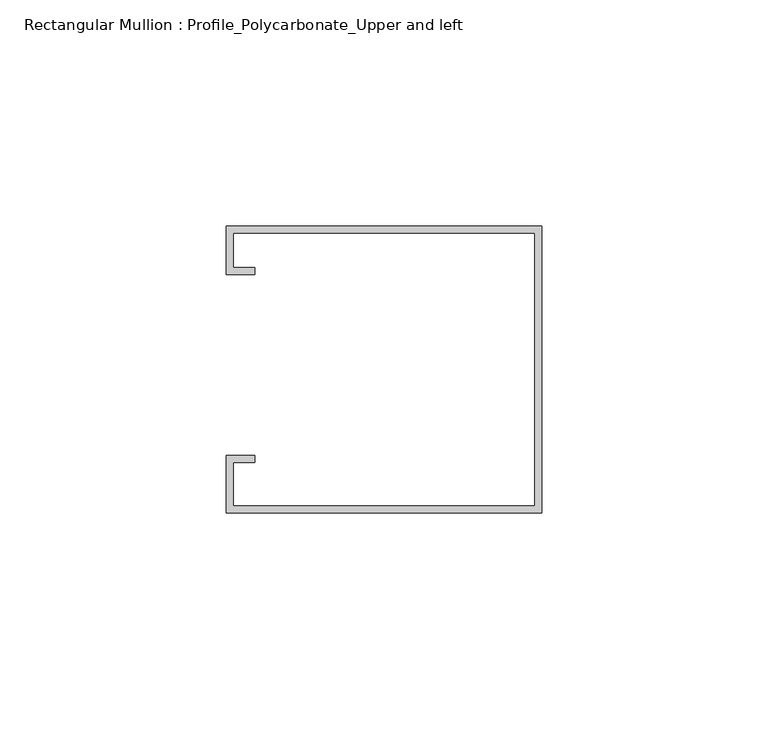
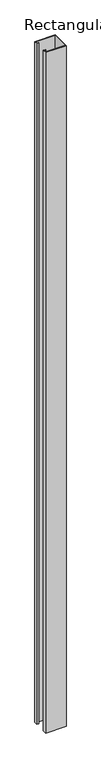
"""IFC4 building model written with IfcOpenShell, lengths in millimetres: member geometry, Rectangular Mullion : Profile_Polycarbonate_Upper and left."""

from ifc_helpers import new_model, si_unit, frame, origin, place, context, project, spatial, polyline, outline, extrude, source, transform, mapped, element, save


def rectangular_mullion_profile_polycarbonate_upper_and_left_a3cdb98e(model_context):
    return source(origin(), model_context, "Body", "SweptSolid", [
        extrude(outline(polyline([(0.0, -32.7), (-69.85, -32.7), (-69.85, -20.0), (-63.5, -20.0), (-63.5, -21.5875), (-68.2625, -21.5875), (-68.2625, -31.1125), (-1.5875, -31.1125), (-1.5875, 29.2125), (-68.2625, 29.2125), (-68.2625, 21.5875), (-63.5, 21.5875), (-63.5, 20.0), (-69.85, 20.0), (-69.85, 30.8), (0.0, 30.8), (0.0, -32.7)])), frame((0.0, 0.0, -2461.6132885), z_axis=(0.0, 0.0, 1.0), x_axis=(1.0, 0.0, 0.0)), (0.0, 0.0, 1.0), 2461.6132885),
    ])


if __name__ == "__main__":
    model = new_model("IFC4")
    model_context = context("Model", 3, world=origin())
    ifc_project = project(units=[si_unit("LENGTHUNIT", "METRE", prefix="MILLI")], contexts=[model_context])
    site = spatial("IfcSite", under=ifc_project)
    building = spatial("IfcBuilding", under=site)
    placement = place(None, origin())
    rectangular_mullion_profile_polycarbonate_upper_and_left_shape = rectangular_mullion_profile_polycarbonate_upper_and_left_a3cdb98e(model_context)
    element("IfcMember", 1, ObjectType="Rectangular Mullion : Profile_Polycarbonate_Upper and left", at=placement, inside=building, context=model_context, shape_type="MappedRepresentation", body=[
        mapped(rectangular_mullion_profile_polycarbonate_upper_and_left_shape, transform((0.0, 0.0, 0.0), x_axis=(1.0, 0.0, 0.0), y_axis=(0.0, 1.0, 0.0), z_axis=(0.0, 0.0, 1.0))),
    ])
    save(model, "model.ifc")

# Revit data of these elements
# Type "Rectangular Mullion : Profile_Polycarbonate_Upper and left"
#   built-in parameter 1007322 = 0.208333 (stored number, unit not read)
#   built-in parameter 1007321 = 0.00520833 (stored number, unit not read)
#   built-in parameter 1007320 = 0 (stored number, unit not read)
# Element 1 (IfcMember, "Rectangular Mullion : Profile_Polycarbonate_Upper and left")
#   Materials on its faces: "ALUMINUM PROFILE AT POLYCARBONATE PANEL"
# Materials
#   "ALUMINUM PROFILE AT POLYCARBONATE PANEL": class "Metal", colour RGB 244 244 244, transparency 0, Description = "Aluminum 6061", Cost = 0
